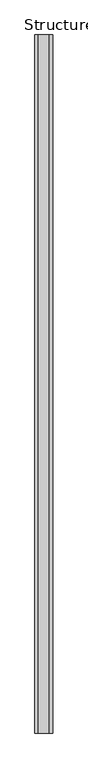
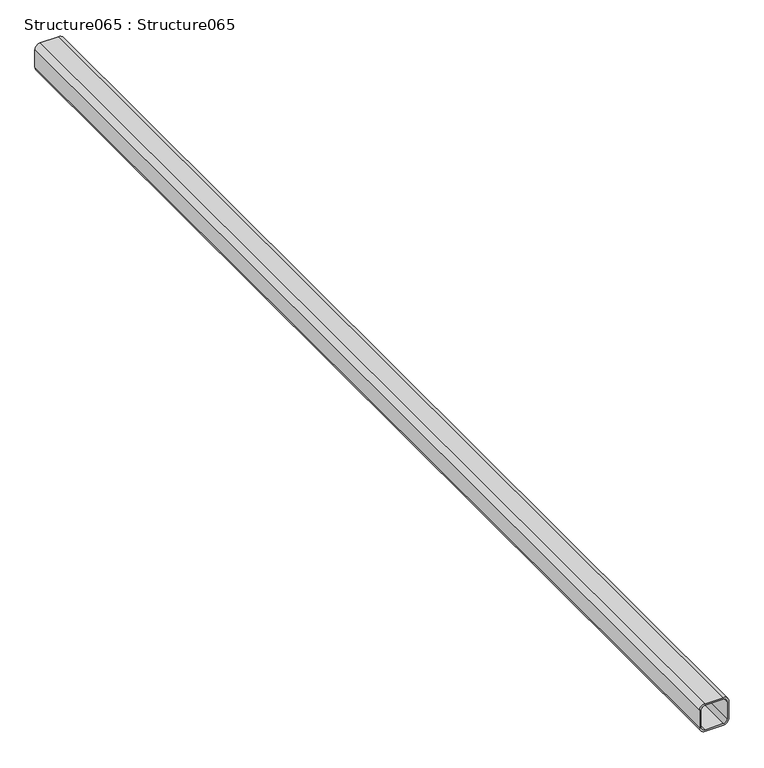
"""IFC4 building model written with IfcOpenShell, lengths in millimetres: proxy geometry, Structure065 : Structure065."""

from ifc_helpers import new_model, si_unit, point, frame, frame_2d, origin, place, context, project, spatial, polyline, circle_curve, trimmed, segment, composite_curve, outline, extrude, source, transform, mapped, element, save


def structure065_structure065_f110fce2(model_context):
    return source(origin(), model_context, "Body", "SweptSolid", [
        extrude(outline(composite_curve([segment(polyline([(40763.5716161, 16355.2668635), (40731.8216161, 16355.2668635)]), True, "CONTINUOUS"), segment(trimmed(circle_curve(frame_2d((40731.8216161, 16364.7918635)), 9.525), [point((40731.8216161, 16355.2668635))], [point((40722.2966161, 16364.7918635))], False, "CARTESIAN"), True, "CONTINUOUS"), segment(polyline([(40722.2966161, 16364.7918635), (40722.2966161, 16396.5418635)]), True, "CONTINUOUS"), segment(trimmed(circle_curve(frame_2d((40731.8216161, 16396.5418635)), 9.525), [point((40722.2966161, 16396.5418635))], [point((40731.8216161, 16406.0668635))], False, "CARTESIAN"), True, "CONTINUOUS"), segment(polyline([(40731.8216161, 16406.0668635), (40763.5716161, 16406.0668635)]), True, "CONTINUOUS"), segment(trimmed(circle_curve(frame_2d((40763.5716161, 16396.5418635)), 9.525), [point((40763.5716161, 16406.0668635))], [point((40773.0966161, 16396.5418635))], False, "CARTESIAN"), True, "CONTINUOUS"), segment(polyline([(40773.0966161, 16396.5418635), (40773.0966161, 16364.7918635)]), True, "CONTINUOUS"), segment(trimmed(circle_curve(frame_2d((40763.5716161, 16364.7918635)), 9.525), [point((40773.0966161, 16364.7918635))], [point((40763.5716161, 16355.2668635))], False, "CARTESIAN"), True, "CONTINUOUS")], self_intersect=False), holes=[composite_curve([segment(polyline([(40731.8216161, 16358.4418635), (40763.5716161, 16358.4418635)]), True, "CONTINUOUS"), segment(trimmed(circle_curve(frame_2d((40763.5716161, 16364.7918635)), 6.35), [point((40763.5716161, 16358.4418635))], [point((40769.9216161, 16364.7918635))], True, "CARTESIAN"), True, "CONTINUOUS"), segment(polyline([(40769.9216161, 16364.7918635), (40769.9216161, 16396.5418635)]), True, "CONTINUOUS"), segment(trimmed(circle_curve(frame_2d((40763.5716161, 16396.5418635)), 6.35), [point((40769.9216161, 16396.5418635))], [point((40763.5716161, 16402.8918635))], True, "CARTESIAN"), True, "CONTINUOUS"), segment(polyline([(40763.5716161, 16402.8918635), (40731.8216161, 16402.8918635)]), True, "CONTINUOUS"), segment(trimmed(circle_curve(frame_2d((40731.8216161, 16396.5418635)), 6.35), [point((40731.8216161, 16402.8918635))], [point((40725.4716161, 16396.5418635))], True, "CARTESIAN"), True, "CONTINUOUS"), segment(polyline([(40725.4716161, 16396.5418635), (40725.4716161, 16364.7918635)]), True, "CONTINUOUS"), segment(trimmed(circle_curve(frame_2d((40731.8216161, 16364.7918635)), 6.35), [point((40725.4716161, 16364.7918635))], [point((40731.8216161, 16358.4418635))], True, "CARTESIAN"), True, "CONTINUOUS")], self_intersect=False)]), frame((0.0, 7982.1449183, 0.0), z_axis=(0.0, 1.0, 0.0), x_axis=(0.0, 0.0, 1.0)), (0.0, 0.0, 1.0), 2000.0),
    ])


if __name__ == "__main__":
    model = new_model("IFC4")
    model_context = context("Model", 3, world=origin())
    ifc_project = project(units=[si_unit("LENGTHUNIT", "METRE", prefix="MILLI")], contexts=[model_context])
    site = spatial("IfcSite", under=ifc_project)
    building = spatial("IfcBuilding", under=site)
    placement = place(None, origin())
    structure065_structure065_shape = structure065_structure065_f110fce2(model_context)
    element("IfcBuildingElementProxy", 1, Name="Structure065 : Structure065", ObjectType="Structure065 : Structure065", at=placement, inside=building, context=model_context, shape_type="MappedRepresentation", body=[
        mapped(structure065_structure065_shape, transform((0.0, 0.0, 0.0), x_axis=(1.0, 0.0, 0.0), y_axis=(0.0, 1.0, 0.0), z_axis=(0.0, 0.0, 1.0))),
    ])
    save(model, "model.ifc")

# Revit data of these elements
# Type "Structure065 : Structure065"
#   NameOverride = "Structure065"
# Element 1 (IfcBuildingElementProxy, "Structure065 : Structure065")
#   Materials on its faces: "STEEL STRUCTURE (SEE STRUCTURAL DWGS)"
# Materials
#   "STEEL STRUCTURE (SEE STRUCTURAL DWGS)": class "Unassigned", colour RGB 128 128 128, transparency 0, Cost = 0
